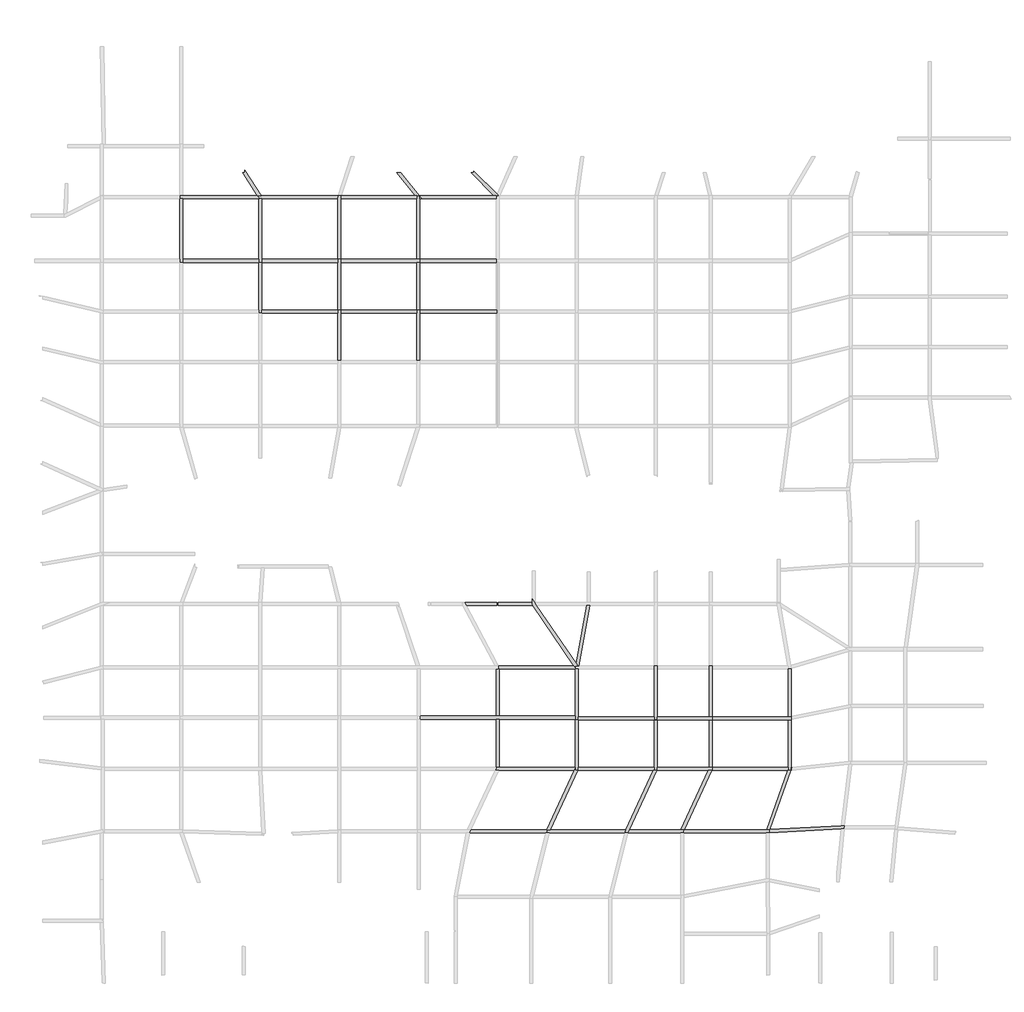
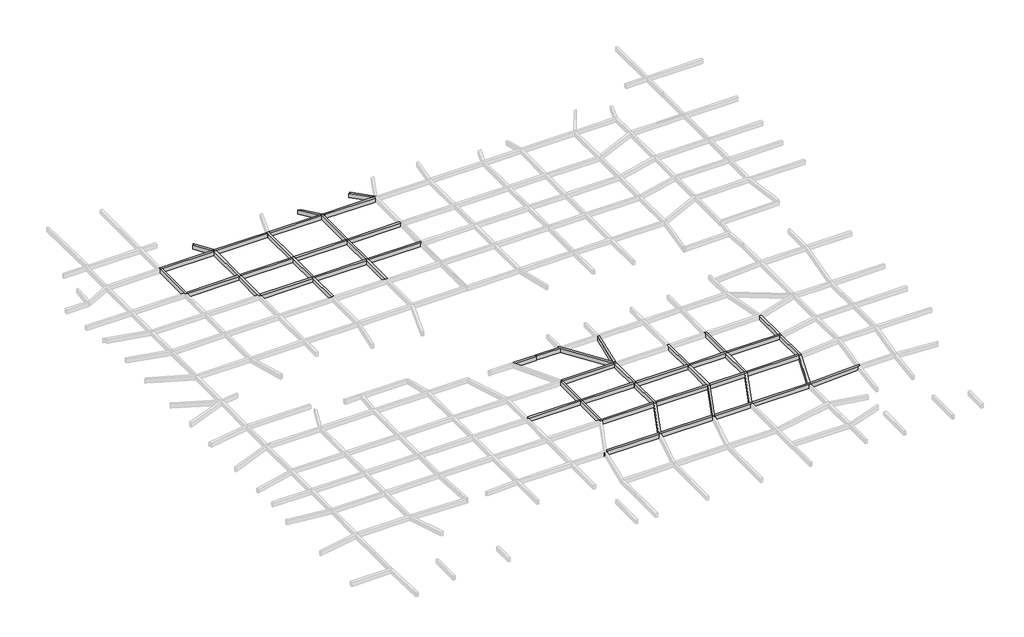
# One storey, part 9 of 15: 54 beams.
"""IFC4 building model written with IfcOpenShell, lengths in millimetres."""

from ifc_helpers import new_model, si_unit, frame, origin, place, context, project, spatial, polyline, outline, extrude, faceted_brep, element, save

model = new_model("IFC4")

# Units and contexts
model_context = context("Model", 3, world=origin())
ifc_project = project(units=[si_unit("LENGTHUNIT", "METRE", prefix="MILLI")], contexts=[model_context])

# Site, building, storey
site = spatial("IfcSite", under=ifc_project)
building = spatial("IfcBuilding", under=site)
storey = spatial("IfcBuildingStorey", under=building, Name="层高", Elevation=3300.0)

# Beams
placement = place(None, origin())
element("IfcBeam", 1, ObjectType="混凝土 - 矩形梁 : KL_beam", at=placement, inside=storey, context=model_context, shape_type="Brep", body=[
    faceted_brep([(208150.3009381, 75092.1684205, 3300.0), (208450.3009381, 75092.1684205, 3300.0), (208450.3009381, 75392.1684205, 3300.0), (208450.3009381, 80084.9176514, 3300.0), (208450.3009381, 80384.9176514, 3300.0), (208150.3009381, 80384.9176514, 3300.0), (208150.3009381, 80092.1684205, 3300.0), (208150.3009381, 75391.5531297, 3300.0), (208150.3009381, 75092.1684205, 2700.0), (208150.3009381, 80384.9176514, 2700.0), (208150.3009381, 80092.1684205, 2700.0), (208150.3009381, 75391.5531297, 2700.0), (208450.3009381, 75092.1684205, 2700.0), (208450.3009381, 80384.9176514, 2700.0), (208450.3009381, 80084.9176514, 2700.0), (208450.3009381, 75392.1684205, 2700.0)], [[[0, 1, 2, 3, 4, 5, 6, 7]], [[8, 0, 7, 6, 5, 9, 10, 11]], [[12, 8, 11, 10, 9, 13, 14, 15]], [[1, 12, 15, 14, 13, 4, 3, 2]], [[1, 0, 8, 12]], [[5, 4, 13, 9]]]),
])
element("IfcBeam", 2, ObjectType="混凝土 - 矩形梁 : KL_beam", at=placement, inside=storey, context=model_context, shape_type="Brep", body=[
    faceted_brep([(213850.3009381, 75092.1684205, 3300.0), (213850.3009381, 75392.1684205, 3300.0), (213550.3009381, 75392.1684205, 3300.0), (208450.3009381, 75392.1684205, 3300.0), (208450.3009381, 75092.1684205, 3300.0), (213549.7300619, 75092.1684205, 3300.0), (213849.7300619, 75092.1684205, 3300.0), (213850.3009381, 75092.1684205, 2700.0), (208450.3009381, 75092.1684205, 2700.0), (213549.7300619, 75092.1684205, 2700.0), (213849.7300619, 75092.1684205, 2700.0), (213850.3009381, 75392.1684205, 2700.0), (208450.3009381, 75392.1684205, 2700.0), (213550.3009381, 75392.1684205, 2700.0)], [[[0, 1, 2, 3, 4, 5, 6]], [[7, 0, 6, 5, 4, 8, 9, 10]], [[11, 7, 10, 9, 8, 12, 13]], [[1, 11, 13, 12, 3, 2]], [[4, 3, 12, 8]], [[1, 0, 7, 11]]]),
])
element("IfcBeam", 3, ObjectType="混凝土 - 矩形梁 : KL_beam", at=placement, inside=storey, context=model_context, shape_type="Brep", body=[
    faceted_brep([(213850.3009381, 80384.9176514, 3300.0), (213550.3009381, 80384.9176514, 3300.0), (213550.3009381, 80084.9176514, 3300.0), (213550.3009381, 75392.1684205, 3300.0), (213850.3009381, 75392.1684205, 3300.0), (213850.3009381, 80092.1684205, 3300.0), (213550.3009381, 80384.9176514, 2700.0), (213550.3009381, 80084.9176514, 2700.0), (213550.3009381, 75392.1684205, 2700.0), (213850.3009381, 80384.9176514, 2700.0), (213850.3009381, 80092.1684205, 2700.0), (213850.3009381, 75392.1684205, 2700.0)], [[[0, 1, 2, 3, 4, 5]], [[1, 6, 7, 8, 3, 2]], [[6, 9, 10, 11, 8, 7]], [[9, 0, 5, 4, 11, 10]], [[4, 3, 8, 11]], [[1, 0, 9, 6]]]),
])
element("IfcBeam", 4, ObjectType="混凝土 - 矩形梁 : KL_beam", at=placement, inside=storey, context=model_context, shape_type="Brep", body=[
    faceted_brep([(200361.325629, 75091.5531297, 3300.0), (200661.325629, 75091.5531297, 3300.0), (200661.325629, 75391.5531297, 3300.0), (200661.325629, 80092.1684205, 3300.0), (200361.325629, 80092.1684205, 3300.0), (200361.325629, 75445.2581831, 3300.0), (200361.325629, 75145.2581831, 3300.0), (200361.325629, 75091.5531297, 2700.0), (200361.325629, 80092.1684205, 2700.0), (200361.325629, 75445.2581831, 2700.0), (200361.325629, 75145.2581831, 2700.0), (200661.325629, 75091.5531297, 2700.0), (200661.325629, 80092.1684205, 2700.0), (200661.325629, 75391.5531297, 2700.0)], [[[0, 1, 2, 3, 4, 5, 6]], [[7, 0, 6, 5, 4, 8, 9, 10]], [[11, 7, 10, 9, 8, 12, 13]], [[1, 11, 13, 12, 3, 2]], [[4, 3, 12, 8]], [[1, 0, 7, 11]]]),
])
element("IfcBeam", 5, ObjectType="混凝土 - 矩形梁 : KL_beam", at=placement, inside=storey, context=model_context, shape_type="Brep", body=[
    faceted_brep([(208450.3009381, 75091.5531297, 3300.0), (208450.3009381, 75092.1684205, 3300.0), (208150.3009381, 75092.1684205, 3300.0), (208150.3009381, 75391.5531297, 3300.0), (200661.325629, 75391.5531297, 3300.0), (200661.325629, 75091.5531297, 3300.0), (208150.3009381, 75091.5531297, 3300.0), (208450.3009381, 75091.5531297, 2700.0), (200661.325629, 75091.5531297, 2700.0), (208150.3009381, 75091.5531297, 2700.0), (208450.3009381, 75092.1684205, 2700.0), (200661.325629, 75391.5531297, 2700.0), (208150.3009381, 75391.5531297, 2700.0), (208150.3009381, 75092.1684205, 2700.0)], [[[0, 1, 2, 3, 4, 5, 6]], [[7, 0, 6, 5, 8, 9]], [[10, 7, 9, 8, 11, 12, 13]], [[3, 12, 11, 4]], [[0, 7, 10, 1]], [[2, 13, 12, 3]], [[13, 2, 1, 10]], [[5, 4, 11, 8]]]),
])
element("IfcBeam", 6, ObjectType="混凝土 - 矩形梁 : KL_beam", at=placement, inside=storey, context=model_context, shape_type="Brep", body=[
    faceted_brep([(208150.3009381, 70090.9378389, 3300.0), (208395.8614772, 70090.9378389, 3300.0), (208450.3009381, 70090.9378389, 3300.0), (208450.3009381, 70390.9378389, 3300.0), (208450.3009381, 75091.5531297, 3300.0), (208150.3009381, 75091.5531297, 3300.0), (208150.3009381, 70390.9378389, 3300.0), (208450.3009381, 70090.9378389, 2700.0), (208450.3009381, 70390.9378389, 2700.0), (208450.3009381, 75091.5531297, 2700.0), (208395.8614772, 70090.9378389, 2700.0), (208150.3009381, 70090.9378389, 2700.0), (208150.3009381, 70390.9378389, 2700.0), (208150.3009381, 75091.5531297, 2700.0)], [[[0, 1, 2, 3, 4, 5, 6]], [[2, 7, 8, 9, 4, 3]], [[7, 10, 11, 12, 13, 9, 8]], [[11, 0, 6, 5, 13, 12]], [[5, 4, 9, 13]], [[2, 1, 0, 11, 10, 7]]]),
])
element("IfcBeam", 7, ObjectType="混凝土 - 矩形梁 : KL_beam", at=placement, inside=storey, context=model_context, shape_type="Brep", body=[
    faceted_brep([(200361.325629, 70090.9378389, 3300.0), (200607.1105063, 70090.9378389, 3300.0), (200661.325629, 70090.9378389, 3300.0), (200661.325629, 70390.9378389, 3300.0), (200661.325629, 75091.5531297, 3300.0), (200361.325629, 75091.5531297, 3300.0), (200361.325629, 70390.9378389, 3300.0), (200361.325629, 70274.0247745, 3300.0), (200361.325629, 70090.9378389, 2700.0), (200361.325629, 75091.5531297, 2700.0), (200361.325629, 70390.9378389, 2700.0), (200361.325629, 70274.0247745, 2700.0), (200661.325629, 70090.9378389, 2700.0), (200607.1105063, 70090.9378389, 2700.0), (200661.325629, 75091.5531297, 2700.0), (200661.325629, 70390.9378389, 2700.0)], [[[0, 1, 2, 3, 4, 5, 6, 7]], [[8, 0, 7, 6, 5, 9, 10, 11]], [[12, 13, 8, 11, 10, 9, 14, 15]], [[2, 12, 15, 14, 4, 3]], [[5, 4, 14, 9]], [[2, 1, 0, 8, 13, 12]]]),
])
element("IfcBeam", 8, ObjectType="混凝土 - 矩形梁 : KL_beam", at=placement, inside=storey, context=model_context, shape_type="Brep", body=[
    faceted_brep([(208150.3009381, 70090.9378389, 3300.0), (208150.3009381, 70390.9378389, 3300.0), (200661.325629, 70390.9378389, 3300.0), (200661.325629, 70090.9378389, 3300.0), (208064.8481015, 70090.9378389, 3300.0), (208150.3009381, 70090.9378389, 2700.0), (200661.325629, 70090.9378389, 2700.0), (208064.8481015, 70090.9378389, 2700.0), (208150.3009381, 70390.9378389, 2700.0), (200661.325629, 70390.9378389, 2700.0)], [[[0, 1, 2, 3, 4]], [[5, 0, 4, 3, 6, 7]], [[8, 5, 7, 6, 9]], [[1, 8, 9, 2]], [[1, 0, 5, 8]], [[3, 2, 9, 6]]]),
])
element("IfcBeam", 9, ObjectType="混凝土 - 矩形梁 : KL_beam", at=placement, inside=storey, context=model_context, shape_type="Brep", body=[
    faceted_brep([(208450.3009381, 70390.9378389, 2700.0), (208450.3009381, 70390.9378389, 3300.0), (213549.7300619, 70390.9378389, 3300.0), (213849.7300619, 70390.9378389, 3300.0), (213849.7300619, 70390.9378389, 2700.0), (213549.7300619, 70390.9378389, 2700.0), (208450.3009381, 70090.9378389, 3300.0), (208450.3009381, 70090.9378389, 2700.0), (213849.7300619, 70092.1684205, 3300.0), (213849.7300619, 70090.9378389, 3300.0), (213849.7300619, 70090.9378389, 2700.0), (213849.7300619, 70092.1684205, 2700.0), (213464.2379642, 70090.9378389, 3300.0), (213794.9360409, 70090.9378389, 3300.0), (213464.2379642, 70090.9378389, 2700.0), (213794.9360409, 70090.9378389, 2700.0)], [[[0, 1, 2, 3, 4, 5]], [[6, 1, 0, 7]], [[3, 8, 9, 10, 11, 4]], [[1, 6, 12, 13, 9, 8, 3, 2]], [[6, 7, 14, 15, 10, 9, 13, 12]], [[7, 0, 5, 4, 11, 10, 15, 14]]]),
])
element("IfcBeam", 10, ObjectType="混凝土 - 矩形梁 : KL_beam", at=placement, inside=storey, context=model_context, shape_type="Brep", body=[
    faceted_brep([(213849.7300619, 75092.1684205, 3300.0), (213549.7300619, 75092.1684205, 3300.0), (213549.7300619, 70390.9378389, 3300.0), (213849.7300619, 70390.9378389, 3300.0), (213849.7300619, 70392.1684205, 3300.0), (213849.7300619, 75092.1684205, 2700.0), (213849.7300619, 70390.9378389, 2700.0), (213849.7300619, 70392.1684205, 2700.0), (213549.7300619, 75092.1684205, 2700.0), (213549.7300619, 70390.9378389, 2700.0)], [[[0, 1, 2, 3, 4]], [[5, 0, 4, 3, 6, 7]], [[8, 5, 7, 6, 9]], [[1, 8, 9, 2]], [[1, 0, 5, 8]], [[3, 2, 9, 6]]]),
])
element("IfcBeam", 11, ObjectType="混凝土 - 矩形梁 : KL_beam", at=placement, inside=storey, context=model_context, shape_type="Brep", body=[
    faceted_brep([(221650.3009384, 75092.1684205, 3300.0), (221650.3009384, 75119.2786858, 3300.0), (221650.3009384, 75392.1684205, 3300.0), (221485.3991695, 75392.1684205, 3300.0), (221350.3009384, 75392.1684205, 3300.0), (213850.3009381, 75392.1684205, 3300.0), (213850.3009381, 75092.1684205, 3300.0), (221350.3009384, 75092.1684205, 3300.0), (221650.3009384, 75092.1684205, 2700.0), (213850.3009381, 75092.1684205, 2700.0), (221350.3009384, 75092.1684205, 2700.0), (221650.3009384, 75392.1684205, 2700.0), (221650.3009384, 75119.2786858, 2700.0), (213850.3009381, 75392.1684205, 2700.0), (221350.3009384, 75392.1684205, 2700.0), (221485.3991695, 75392.1684205, 2700.0)], [[[0, 1, 2, 3, 4, 5, 6, 7]], [[8, 0, 7, 6, 9, 10]], [[11, 12, 8, 10, 9, 13, 14, 15]], [[2, 11, 15, 14, 13, 5, 4, 3]], [[6, 5, 13, 9]], [[2, 1, 0, 8, 12, 11]]]),
])
element("IfcBeam", 12, ObjectType="混凝土 - 矩形梁 : KL_beam", at=placement, inside=storey, context=model_context, shape_type="Brep", body=[
    faceted_brep([(221350.3009384, 70092.1684205, 3300.0), (221606.4676056, 70092.1684205, 3300.0), (221650.3009384, 70092.1684205, 3300.0), (221650.3009384, 70106.4638205, 3300.0), (221650.3009384, 70216.5015374, 3300.0), (221650.3009384, 70407.9697272, 3300.0), (221650.3009384, 75092.1684205, 3300.0), (221350.3009384, 75092.1684205, 3300.0), (221350.3009384, 70392.1684205, 3300.0), (221350.3009384, 70092.1684205, 2700.0), (221350.3009384, 75092.1684205, 2700.0), (221350.3009384, 70392.1684205, 2700.0), (221650.3009384, 70092.1684205, 2700.0), (221606.4676056, 70092.1684205, 2700.0), (221650.3009384, 75092.1684205, 2700.0), (221650.3009384, 70407.9697272, 2700.0), (221650.3009384, 70216.5015374, 2700.0), (221650.3009384, 70106.4638205, 2700.0)], [[[0, 1, 2, 3, 4, 5, 6, 7, 8]], [[9, 0, 8, 7, 10, 11]], [[12, 13, 9, 11, 10, 14, 15, 16, 17]], [[2, 12, 17, 16, 15, 14, 6, 5, 4, 3]], [[7, 6, 14, 10]], [[2, 1, 0, 9, 13, 12]]]),
])
element("IfcBeam", 13, ObjectType="混凝土 - 矩形梁 : KL_beam", at=placement, inside=storey, context=model_context, shape_type="Brep", body=[
    faceted_brep([(213849.7300619, 70392.1684205, 3300.0), (213849.7300619, 70390.9378389, 3300.0), (213849.7300619, 70092.1684205, 3300.0), (221288.3700133, 70092.1684205, 3300.0), (221350.3009384, 70092.1684205, 3300.0), (221350.3009384, 70392.1684205, 3300.0), (213849.7300619, 70392.1684205, 2700.0), (221350.3009384, 70392.1684205, 2700.0), (213849.7300619, 70092.1684205, 2700.0), (213849.7300619, 70390.9378389, 2700.0), (221350.3009384, 70092.1684205, 2700.0), (221288.3700133, 70092.1684205, 2700.0)], [[[0, 1, 2, 3, 4, 5]], [[6, 0, 5, 7]], [[8, 9, 6, 7, 10, 11]], [[2, 8, 11, 10, 4, 3]], [[8, 2, 1, 0, 6, 9]], [[5, 4, 10, 7]]]),
])
element("IfcBeam", 14, ObjectType="混凝土 - 矩形梁 : KL_beam", at=placement, inside=storey, context=model_context, shape_type="Brep", body=[
    faceted_brep([(205522.0572974, 63928.0448871, 3300.0), (205661.9495948, 64228.0448871, 3300.0), (208395.8614772, 70090.9378389, 3300.0), (208150.3009381, 70090.9378389, 3300.0), (208064.8481015, 70090.9378389, 3300.0), (205337.522131, 64242.1684205, 3300.0), (205250.1649613, 64054.8303656, 3300.0), (205491.7692821, 63942.1684205, 3300.0), (208064.8481015, 70090.9378389, 2700.0), (205337.522131, 64242.1684205, 2700.0), (205250.1649613, 64054.8303656, 2700.0), (208395.8614772, 70090.9378389, 2700.0), (205661.9495948, 64228.0448871, 2700.0), (205522.0572974, 63928.0448871, 2700.0), (205491.7692821, 63942.1684205, 2700.0), (208150.3009381, 70090.9378389, 2700.0)], [[[0, 1, 2, 3, 4, 5, 6, 7]], [[6, 5, 4, 8, 9, 10]], [[11, 12, 13, 14, 10, 9, 8, 15]], [[2, 1, 0, 13, 12, 11]], [[2, 11, 15, 8, 4, 3]], [[0, 7, 6, 10, 14, 13]]]),
])
element("IfcBeam", 15, ObjectType="混凝土 - 矩形梁 : KL_beam", at=placement, inside=storey, context=model_context, shape_type="Brep", body=[
    faceted_brep([(210936.491926, 63928.0448871, 3300.0), (210945.3598239, 63947.1643462, 3300.0), (211075.6365195, 64228.0448871, 3300.0), (210744.9384428, 64228.0448871, 3300.0), (205661.9495948, 64228.0448871, 3300.0), (205522.0572974, 63928.0448871, 3300.0), (205546.7541217, 63928.0448871, 3300.0), (210741.9011747, 63928.0448871, 3300.0), (210936.491926, 63928.0448871, 2700.0), (205522.0572974, 63928.0448871, 2700.0), (205546.7541217, 63928.0448871, 2700.0), (210741.9011747, 63928.0448871, 2700.0), (211075.6365195, 64228.0448871, 2700.0), (210945.3598239, 63947.1643462, 2700.0), (205661.9495948, 64228.0448871, 2700.0), (210744.9384428, 64228.0448871, 2700.0)], [[[0, 1, 2, 3, 4, 5, 6, 7]], [[8, 0, 7, 6, 5, 9, 10, 11]], [[12, 13, 8, 11, 10, 9, 14, 15]], [[2, 12, 15, 14, 4, 3]], [[5, 4, 14, 9]], [[2, 1, 0, 8, 13, 12]]]),
])
element("IfcBeam", 16, ObjectType="混凝土 - 矩形梁 : KL_beam", at=placement, inside=storey, context=model_context, shape_type="Brep", body=[
    faceted_brep([(210744.9384428, 64228.0448871, 3300.0), (211075.6365195, 64228.0448871, 3300.0), (211084.5044173, 64247.1643462, 3300.0), (213794.9360409, 70090.9378389, 3300.0), (213464.2379642, 70090.9378389, 3300.0), (211075.6365195, 64228.0448871, 2700.0), (211084.5044173, 64247.1643462, 2700.0), (213794.9360409, 70090.9378389, 2700.0), (210744.9384428, 64228.0448871, 2700.0), (213464.2379642, 70090.9378389, 2700.0)], [[[0, 1, 2, 3, 4]], [[1, 5, 6, 7, 3, 2]], [[5, 8, 9, 7, 6]], [[8, 0, 4, 9]], [[1, 0, 8, 5]], [[3, 7, 9, 4]]]),
])
element("IfcBeam", 17, ObjectType="混凝土 - 矩形梁 : KL_beam", at=placement, inside=storey, context=model_context, shape_type="Brep", body=[
    faceted_brep([(211084.5044173, 64247.1643462, 3300.0), (211075.6365195, 64228.0448871, 3300.0), (210945.3598239, 63947.1643462, 3300.0), (211041.9011747, 63947.1643462, 3300.0), (219183.8949524, 63947.1643462, 3300.0), (219483.8949524, 63947.1643462, 3300.0), (219483.8949524, 63954.8196612, 3300.0), (219483.8949524, 64247.1643462, 3300.0), (219329.9670642, 64247.1643462, 3300.0), (219227.7282852, 64247.1643462, 3300.0), (219483.8949524, 64247.1643462, 2700.0), (219329.9670642, 64247.1643462, 2700.0), (219227.7282852, 64247.1643462, 2700.0), (211084.5044173, 64247.1643462, 2700.0), (210945.3598239, 63947.1643462, 2700.0), (211075.6365195, 64228.0448871, 2700.0), (219483.8949524, 63954.8196612, 2700.0), (219483.8949524, 63947.1643462, 2700.0), (219183.8949524, 63947.1643462, 2700.0), (211041.9011747, 63947.1643462, 2700.0)], [[[0, 1, 2, 3, 4, 5, 6, 7, 8, 9]], [[7, 10, 11, 12, 13, 0, 9, 8]], [[14, 15, 13, 12, 11, 10, 16, 17, 18, 19]], [[2, 14, 19, 18, 17, 5, 4, 3]], [[0, 13, 15, 14, 2, 1]], [[7, 6, 5, 17, 16, 10]]]),
])
element("IfcBeam", 18, ObjectType="混凝土 - 矩形梁 : KL_beam", at=placement, inside=storey, context=model_context, shape_type="Brep", body=[
    faceted_brep([(205337.522131, 64242.1684205, 3300.0), (197894.9093254, 64242.1684205, 3300.0), (197564.2230667, 64242.1684205, 3300.0), (197564.2230667, 63942.1684205, 3300.0), (197777.200788, 63942.1684205, 3300.0), (205241.0914253, 63942.1684205, 3300.0), (205491.7692821, 63942.1684205, 3300.0), (205250.1649613, 64054.8303656, 3300.0), (205330.9362192, 64228.0448871, 3300.0), (197564.2230667, 63942.1684205, 2700.0), (197777.200788, 63942.1684205, 2700.0), (205241.0914253, 63942.1684205, 2700.0), (205491.7692821, 63942.1684205, 2700.0), (197564.2230667, 64242.1684205, 2700.0), (197894.9093254, 64242.1684205, 2700.0), (205337.522131, 64242.1684205, 2700.0), (205330.9362192, 64228.0448871, 2700.0), (205250.1649613, 64054.8303656, 2700.0)], [[[0, 1, 2, 3, 4, 5, 6, 7, 8]], [[6, 5, 4, 3, 9, 10, 11, 12]], [[12, 11, 10, 9, 13, 14, 15, 16, 17]], [[2, 1, 0, 15, 14, 13]], [[7, 17, 16, 15, 0, 8]], [[17, 7, 6, 12]], [[2, 13, 9, 3]]]),
])
element("IfcBeam", 19, ObjectType="混凝土 - 矩形梁 : KL_beam", at=placement, inside=storey, context=model_context, shape_type="Brep", body=[
    faceted_brep([(200361.325629, 70274.0247745, 3300.0), (200276.4242476, 70090.9378389, 3300.0), (197564.2230667, 64242.1684205, 3300.0), (197894.9093254, 64242.1684205, 3300.0), (200607.1105063, 70090.9378389, 3300.0), (200361.325629, 70090.9378389, 3300.0), (200361.325629, 70274.0247745, 2700.0), (200276.4242476, 70090.9378389, 2700.0), (197564.2230667, 64242.1684205, 2700.0), (200361.325629, 70090.9378389, 2700.0), (200607.1105063, 70090.9378389, 2700.0), (197894.9093254, 64242.1684205, 2700.0)], [[[0, 1, 2, 3, 4, 5]], [[2, 1, 0, 6, 7, 8]], [[8, 7, 6, 9, 10, 11]], [[10, 4, 3, 11]], [[5, 9, 6, 0]], [[9, 5, 4, 10]], [[3, 2, 8, 11]]]),
])
element("IfcBeam", 20, ObjectType="混凝土 - 矩形梁 : KL_beam", at=placement, inside=storey, context=model_context, shape_type="Brep", body=[
    faceted_brep([(192604.8334695, 70390.9378389, 3300.0), (192464.0250307, 70090.9378389, 3300.0), (192795.4266246, 70090.9378389, 3300.0), (200276.4242476, 70090.9378389, 3300.0), (200361.325629, 70274.0247745, 3300.0), (200361.325629, 70390.9378389, 3300.0), (192850.1300471, 70390.9378389, 3300.0), (200361.325629, 70390.9378389, 2700.0), (192850.1300471, 70390.9378389, 2700.0), (192604.8334695, 70390.9378389, 2700.0), (192464.0250307, 70090.9378389, 2700.0), (200361.325629, 70274.0247745, 2700.0), (200276.4242476, 70090.9378389, 2700.0), (192795.4266246, 70090.9378389, 2700.0)], [[[0, 1, 2, 3, 4, 5, 6]], [[5, 7, 8, 9, 0, 6]], [[10, 9, 8, 7, 11, 12, 13]], [[1, 10, 13, 12, 3, 2]], [[7, 5, 4, 11]], [[4, 3, 12, 11]], [[1, 0, 9, 10]]]),
])
element("IfcBeam", 21, ObjectType="混凝土 - 矩形梁 : KL_beam", at=placement, inside=storey, context=model_context, shape_type="Brep", body=[
    faceted_brep([(189578.0296218, 63942.1684205, 3300.0), (189632.1700876, 63942.1684205, 3300.0), (189937.7850961, 63942.1684205, 3300.0), (197468.0166992, 63942.1684205, 3300.0), (197564.2230667, 63942.1684205, 3300.0), (197564.2230667, 64242.1684205, 3300.0), (190050.2396546, 64242.1684205, 3300.0), (189910.8814312, 63945.2581831, 3300.0), (189579.4798373, 63945.2581831, 3300.0), (197564.2230667, 64242.1684205, 2700.0), (190050.2396546, 64242.1684205, 2700.0), (197564.2230667, 63942.1684205, 2700.0), (197468.0166992, 63942.1684205, 2700.0), (189937.7850961, 63942.1684205, 2700.0), (189632.1700876, 63942.1684205, 2700.0), (189578.0296218, 63942.1684205, 2700.0), (189579.4798373, 63945.2581831, 2700.0), (189910.8814312, 63945.2581831, 2700.0)], [[[0, 1, 2, 3, 4, 5, 6, 7, 8]], [[5, 9, 10, 6]], [[11, 12, 13, 14, 15, 16, 17, 10, 9]], [[0, 15, 14, 13, 12, 11, 4, 3, 2, 1]], [[15, 0, 8, 16]], [[5, 4, 11, 9]], [[7, 17, 16, 8]], [[17, 7, 6, 10]]]),
])
element("IfcBeam", 22, ObjectType="混凝土 - 矩形梁 : KL_beam", at=placement, inside=storey, context=model_context, shape_type="Brep", body=[
    faceted_brep([(185065.5848537, 75445.2581831, 3300.0), (185065.5848537, 75145.2581831, 3300.0), (192550.1300471, 75145.2581831, 3300.0), (192850.1300471, 75145.2581831, 3300.0), (200361.325629, 75145.2581831, 3300.0), (200361.325629, 75445.2581831, 3300.0), (192850.1300471, 75445.2581831, 3300.0), (192550.1300471, 75445.2581831, 3300.0), (185065.5848537, 75145.2581831, 2700.0), (192550.1300471, 75145.2581831, 2700.0), (192850.1300471, 75145.2581831, 2700.0), (200361.325629, 75145.2581831, 2700.0), (185065.5848537, 75445.2581831, 2700.0), (192550.1300471, 75445.2581831, 2700.0), (192850.1300471, 75445.2581831, 2700.0), (200361.325629, 75445.2581831, 2700.0)], [[[0, 1, 2, 3, 4, 5, 6, 7]], [[1, 8, 9, 10, 11, 4, 3, 2]], [[8, 12, 13, 14, 15, 11, 10, 9]], [[12, 0, 7, 6, 5, 15, 14, 13]], [[1, 0, 12, 8]], [[5, 4, 11, 15]]]),
])
element("IfcBeam", 23, ObjectType="混凝土 - 矩形梁 : KL_beam", at=placement, inside=storey, context=model_context, shape_type="Brep", body=[
    faceted_brep([(200361.325629, 80392.1684205, 3300.0), (200590.9130323, 80392.1684205, 3300.0), (200430.7160379, 80628.7721233, 3300.0), (196535.9381364, 86381.1826239, 3300.0), (196428.3344611, 86540.1083772, 3300.0), (196128.3344611, 86983.1947852, 3300.0), (196128.3344611, 86681.1826239, 3300.0), (196128.3344611, 86448.1008075, 3300.0), (196173.642678, 86381.1826239, 3300.0), (200228.6175739, 80392.1684205, 3300.0), (200361.325629, 80196.1646357, 3300.0), (200361.325629, 80196.1646357, 2700.0), (196128.3344611, 86448.1008075, 2700.0), (196173.642678, 86381.1826239, 2700.0), (200228.6175739, 80392.1684205, 2700.0), (200590.9130323, 80392.1684205, 2700.0), (200361.325629, 80392.1684205, 2700.0), (196128.3344611, 86681.1826239, 2700.0), (196128.3344611, 86983.1947852, 2700.0), (196428.3344611, 86540.1083772, 2700.0), (196535.9381364, 86381.1826239, 2700.0), (200430.7160379, 80628.7721233, 2700.0)], [[[0, 1, 2, 3, 4, 5, 6, 7, 8, 9, 10]], [[11, 10, 9, 8, 7, 12, 13, 14]], [[15, 16, 11, 14, 13, 12, 17, 18, 19, 20, 21]], [[1, 15, 21, 20, 19, 18, 5, 4, 3, 2]], [[0, 16, 15, 1]], [[16, 0, 10, 11]], [[7, 6, 5, 18, 17, 12]]]),
])
element("IfcBeam", 24, ObjectType="混凝土 - 矩形梁 : KL_beam", at=placement, inside=storey, context=model_context, shape_type="Brep", body=[
    faceted_brep([(200361.325629, 80092.1684205, 3300.0), (200361.325629, 80196.1646357, 3300.0), (200228.6175739, 80392.1684205, 3300.0), (192790.538789, 80392.1684205, 3300.0), (192790.538789, 80092.1684205, 3300.0), (192850.1300471, 80092.1684205, 3300.0), (200228.6175739, 80392.1684205, 2700.0), (192790.538789, 80392.1684205, 2700.0), (200361.325629, 80196.1646357, 2700.0), (200361.325629, 80092.1684205, 2700.0), (192850.1300471, 80092.1684205, 2700.0), (192790.538789, 80092.1684205, 2700.0)], [[[0, 1, 2, 3, 4, 5]], [[2, 6, 7, 3]], [[8, 9, 10, 11, 7, 6]], [[9, 0, 5, 4, 11, 10]], [[0, 9, 8, 1]], [[2, 1, 8, 6]], [[4, 3, 7, 11]]]),
])
element("IfcBeam", 25, ObjectType="混凝土 - 矩形梁 : KL_beam", at=placement, inside=storey, context=model_context, shape_type="Brep", body=[
    faceted_brep([(185050.3009381, 115492.1448334, 3300.0), (184750.3009381, 115492.1448334, 3300.0), (184750.3009381, 115192.1448334, 3300.0), (184750.3009381, 110492.1448334, 3300.0), (185050.3009381, 110492.1448334, 3300.0), (185050.3009381, 115192.1448334, 3300.0), (184750.3009381, 115492.1448334, 2700.0), (184750.3009381, 115192.1448334, 2700.0), (184750.3009381, 110492.1448334, 2700.0), (185050.3009381, 115492.1448334, 2700.0), (185050.3009381, 115192.1448334, 2700.0), (185050.3009381, 110492.1448334, 2700.0)], [[[0, 1, 2, 3, 4, 5]], [[1, 6, 7, 8, 3, 2]], [[6, 9, 10, 11, 8, 7]], [[9, 0, 5, 4, 11, 10]], [[4, 3, 8, 11]], [[1, 0, 9, 6]]]),
])
element("IfcBeam", 26, ObjectType="混凝土 - 矩形梁 : KL_beam", at=placement, inside=storey, context=model_context, shape_type="Brep", body=[
    faceted_brep([(177250.3009381, 115492.1448334, 3300.0), (176950.3009381, 115492.1448334, 3300.0), (176950.3009381, 115192.1448334, 3300.0), (176950.3009381, 110492.1448334, 3300.0), (177250.3009381, 110492.1448334, 3300.0), (177250.3009381, 115192.1448334, 3300.0), (176950.3009381, 115492.1448334, 2700.0), (176950.3009381, 115192.1448334, 2700.0), (176950.3009381, 110492.1448334, 2700.0), (177250.3009381, 115492.1448334, 2700.0), (177250.3009381, 115192.1448334, 2700.0), (177250.3009381, 110492.1448334, 2700.0)], [[[0, 1, 2, 3, 4, 5]], [[1, 6, 7, 8, 3, 2]], [[6, 9, 10, 11, 8, 7]], [[9, 0, 5, 4, 11, 10]], [[4, 3, 8, 11]], [[1, 0, 9, 6]]]),
])
element("IfcBeam", 27, ObjectType="混凝土 - 矩形梁 : KL_beam", at=placement, inside=storey, context=model_context, shape_type="SweptSolid", body=[
    extrude(outline(polyline([(184750.3009381, 115492.1448334), (184750.3009381, 115192.1448334), (177250.3009381, 115192.1448334), (177250.3009381, 115492.1448334), (184750.3009381, 115492.1448334)])), frame((0.0, 0.0, 2700.0), z_axis=(0.0, 0.0, 1.0), x_axis=(1.0, 0.0, 0.0)), (0.0, 0.0, 1.0), 600.0),
])
element("IfcBeam", 28, ObjectType="混凝土 - 矩形梁 : KL_beam", at=placement, inside=storey, context=model_context, shape_type="Brep", body=[
    faceted_brep([(177250.3009381, 120492.1448334, 3300.0), (176950.3009381, 120492.1448334, 3300.0), (176950.3009381, 120192.1448334, 3300.0), (176950.3009381, 115492.1448334, 3300.0), (177250.3009381, 115492.1448334, 3300.0), (177250.3009381, 120192.1448334, 3300.0), (176950.3009381, 120492.1448334, 2700.0), (176950.3009381, 120192.1448334, 2700.0), (176950.3009381, 115492.1448334, 2700.0), (177250.3009381, 120492.1448334, 2700.0), (177250.3009381, 120192.1448334, 2700.0), (177250.3009381, 115492.1448334, 2700.0)], [[[0, 1, 2, 3, 4, 5]], [[1, 6, 7, 8, 3, 2]], [[6, 9, 10, 11, 8, 7]], [[9, 0, 5, 4, 11, 10]], [[4, 3, 8, 11]], [[1, 0, 9, 6]]]),
])
element("IfcBeam", 29, ObjectType="混凝土 - 矩形梁 : KL_beam", at=placement, inside=storey, context=model_context, shape_type="Brep", body=[
    faceted_brep([(185050.3009381, 120192.1448334, 3300.0), (185050.3009381, 120492.1448334, 3300.0), (184750.3009381, 120492.1448334, 3300.0), (177250.3009381, 120492.1448334, 3300.0), (177250.3009381, 120192.1448334, 3300.0), (184750.3009381, 120192.1448334, 3300.0), (185050.3009381, 120192.1448334, 2700.0), (177250.3009381, 120192.1448334, 2700.0), (184750.3009381, 120192.1448334, 2700.0), (185050.3009381, 120492.1448334, 2700.0), (177250.3009381, 120492.1448334, 2700.0), (184750.3009381, 120492.1448334, 2700.0)], [[[0, 1, 2, 3, 4, 5]], [[6, 0, 5, 4, 7, 8]], [[9, 6, 8, 7, 10, 11]], [[1, 9, 11, 10, 3, 2]], [[4, 3, 10, 7]], [[1, 0, 6, 9]]]),
])
element("IfcBeam", 30, ObjectType="混凝土 - 矩形梁 : KL_beam", at=placement, inside=storey, context=model_context, shape_type="SweptSolid", body=[
    extrude(outline(polyline([(185050.3009381, 115492.1448334), (184750.3009381, 115492.1448334), (184750.3009381, 120192.1448334), (185050.3009381, 120192.1448334), (185050.3009381, 115492.1448334)])), frame((0.0, 0.0, 2700.0), z_axis=(0.0, 0.0, 1.0), x_axis=(1.0, 0.0, 0.0)), (0.0, 0.0, 1.0), 600.0),
])
element("IfcBeam", 31, ObjectType="混凝土 - 矩形梁 : KL_beam", at=placement, inside=storey, context=model_context, shape_type="Brep", body=[
    faceted_brep([(177250.3009381, 126792.1448334, 3300.0), (176991.4064824, 126792.1448334, 3300.0), (176950.3009381, 126792.1448334, 3300.0), (176950.3009381, 126665.9608383, 3300.0), (176950.3009381, 126492.1448334, 3300.0), (176950.3009381, 120492.1448334, 3300.0), (177250.3009381, 120492.1448334, 3300.0), (177250.3009381, 126492.1448334, 3300.0), (176950.3009381, 126792.1448334, 2700.0), (176950.3009381, 126665.9608383, 2700.0), (176950.3009381, 126492.1448334, 2700.0), (176950.3009381, 120492.1448334, 2700.0), (176991.4064824, 126792.1448334, 2700.0), (177250.3009381, 126792.1448334, 2700.0), (177250.3009381, 126492.1448334, 2700.0), (177250.3009381, 120492.1448334, 2700.0)], [[[0, 1, 2, 3, 4, 5, 6, 7]], [[2, 8, 9, 10, 11, 5, 4, 3]], [[8, 12, 13, 14, 15, 11, 10, 9]], [[13, 0, 7, 6, 15, 14]], [[6, 5, 11, 15]], [[2, 1, 0, 13, 12, 8]]]),
])
element("IfcBeam", 32, ObjectType="混凝土 - 矩形梁 : KL_beam", at=placement, inside=storey, context=model_context, shape_type="Brep", body=[
    faceted_brep([(185050.3009381, 126792.1448334, 3300.0), (184971.847268, 126792.1448334, 3300.0), (184750.3009381, 126792.1448334, 3300.0), (184750.3009381, 126492.1448334, 3300.0), (184750.3009381, 120492.1448334, 3300.0), (185050.3009381, 120492.1448334, 3300.0), (185050.3009381, 126492.1448334, 3300.0), (185050.3009381, 126695.2626192, 3300.0), (184750.3009381, 126792.1448334, 2700.0), (184750.3009381, 126492.1448334, 2700.0), (184750.3009381, 120492.1448334, 2700.0), (184971.847268, 126792.1448334, 2700.0), (185050.3009381, 126792.1448334, 2700.0), (185050.3009381, 126695.2626192, 2700.0), (185050.3009381, 126492.1448334, 2700.0), (185050.3009381, 120492.1448334, 2700.0)], [[[0, 1, 2, 3, 4, 5, 6, 7]], [[2, 8, 9, 10, 4, 3]], [[8, 11, 12, 13, 14, 15, 10, 9]], [[12, 0, 7, 6, 5, 15, 14, 13]], [[5, 4, 10, 15]], [[2, 1, 0, 12, 11, 8]]]),
])
element("IfcBeam", 33, ObjectType="混凝土 - 矩形梁 : KL_beam", at=placement, inside=storey, context=model_context, shape_type="Brep", body=[
    faceted_brep([(177250.3009381, 126792.1448334, 3300.0), (177250.3009381, 126492.1448334, 3300.0), (184750.3009381, 126492.1448334, 3300.0), (184750.3009381, 126792.1448334, 3300.0), (184585.8193983, 126792.1448334, 3300.0), (177306.9230278, 126792.1448334, 3300.0), (177250.3009381, 126492.1448334, 2700.0), (184750.3009381, 126492.1448334, 2700.0), (177250.3009381, 126792.1448334, 2700.0), (177306.9230278, 126792.1448334, 2700.0), (184585.8193983, 126792.1448334, 2700.0), (184750.3009381, 126792.1448334, 2700.0)], [[[0, 1, 2, 3, 4, 5]], [[1, 6, 7, 2]], [[6, 8, 9, 10, 11, 7]], [[8, 0, 5, 4, 3, 11, 10, 9]], [[1, 0, 8, 6]], [[3, 2, 7, 11]]]),
])
element("IfcBeam", 34, ObjectType="混凝土 - 矩形梁 : KL_beam", at=placement, inside=storey, context=model_context, shape_type="Brep", body=[
    faceted_brep([(183161.6670249, 129027.5312684, 3300.0), (182775.6391551, 129027.5312684, 3300.0), (184585.8193983, 126792.1448334, 3300.0), (184750.3009381, 126792.1448334, 3300.0), (184971.847268, 126792.1448334, 3300.0), (183161.6670249, 129027.5312684, 2700.0), (184971.847268, 126792.1448334, 2700.0), (182775.6391551, 129027.5312684, 2700.0), (184750.3009381, 126792.1448334, 2700.0), (184585.8193983, 126792.1448334, 2700.0)], [[[0, 1, 2, 3, 4]], [[5, 0, 4, 6]], [[7, 5, 6, 8, 9]], [[1, 7, 9, 2]], [[1, 0, 5, 7]], [[2, 9, 8, 6, 4, 3]]]),
    faceted_brep([(185050.3009381, 126492.1448334, 3300.0), (185050.3009381, 126695.2626192, 3300.0), (185050.3009381, 126695.2626192, 2700.0), (185050.3009381, 126492.1448334, 2700.0), (185214.782478, 126492.1448334, 2700.0), (185214.782478, 126492.1448334, 3300.0)], [[[0, 1, 2, 3]], [[4, 5, 0, 3]], [[5, 1, 0]], [[1, 5, 4, 2]], [[2, 4, 3]]]),
])
element("IfcBeam", 35, ObjectType="混凝土 - 矩形梁 : KL_beam", at=placement, inside=storey, context=model_context, shape_type="Brep", body=[
    faceted_brep([(169022.9398412, 126792.1448334, 3300.0), (169219.1792514, 126492.1448334, 3300.0), (169450.3009381, 126492.1448334, 3300.0), (176893.6788484, 126492.1448334, 3300.0), (176950.3009381, 126665.9608383, 3300.0), (176950.3009381, 126792.1448334, 3300.0), (169381.4226248, 126792.1448334, 3300.0), (169219.1792514, 126492.1448334, 2700.0), (169450.3009381, 126492.1448334, 2700.0), (176893.6788484, 126492.1448334, 2700.0), (169022.9398412, 126792.1448334, 2700.0), (169381.4226248, 126792.1448334, 2700.0), (176950.3009381, 126792.1448334, 2700.0), (176950.3009381, 126665.9608383, 2700.0)], [[[0, 1, 2, 3, 4, 5, 6]], [[1, 7, 8, 9, 3, 2]], [[7, 10, 11, 12, 13, 9, 8]], [[5, 12, 11, 10, 0, 6]], [[12, 5, 4, 13]], [[4, 3, 9, 13]], [[1, 0, 10, 7]]]),
])
element("IfcBeam", 36, ObjectType="混凝土 - 矩形梁 : KL_beam", at=placement, inside=storey, context=model_context, shape_type="SweptSolid", body=[
    extrude(outline(polyline([(167560.7034552, 129027.5312684), (167760.6969649, 129027.5312684), (167760.6969649, 129269.8209394), (169381.4226248, 126792.1448334), (169022.9398412, 126792.1448334), (167560.7034552, 129027.5312684)])), frame((0.0, 0.0, 2700.0), z_axis=(0.0, 0.0, 1.0), x_axis=(1.0, 0.0, 0.0)), (0.0, 0.0, 1.0), 600.0),
])
element("IfcBeam", 37, ObjectType="混凝土 - 矩形梁 : KL_beam", at=placement, inside=storey, context=model_context, shape_type="Brep", body=[
    faceted_brep([(169219.1792514, 126492.1448334, 3300.0), (169022.9398412, 126792.1448334, 3300.0), (161650.3009383, 126792.1448334, 3300.0), (161350.3009383, 126792.1448334, 3300.0), (161350.3009383, 126492.1448334, 3300.0), (161650.3009383, 126492.1448334, 3300.0), (169150.3009381, 126492.1448334, 3300.0), (169219.1792514, 126492.1448334, 2700.0), (161350.3009383, 126492.1448334, 2700.0), (161650.3009383, 126492.1448334, 2700.0), (169150.3009381, 126492.1448334, 2700.0), (169022.9398412, 126792.1448334, 2700.0), (161350.3009383, 126792.1448334, 2700.0), (161650.3009383, 126792.1448334, 2700.0)], [[[0, 1, 2, 3, 4, 5, 6]], [[7, 0, 6, 5, 4, 8, 9, 10]], [[11, 7, 10, 9, 8, 12, 13]], [[1, 11, 13, 12, 3, 2]], [[1, 0, 7, 11]], [[4, 3, 12, 8]]]),
])
element("IfcBeam", 38, ObjectType="混凝土 - 矩形梁 : KL_beam", at=placement, inside=storey, context=model_context, shape_type="Brep", body=[
    faceted_brep([(161350.3009383, 120192.1448334, 3300.0), (161650.3009383, 120192.1448334, 3300.0), (161650.3009383, 120492.1448334, 3300.0), (161650.3009383, 126492.1448334, 3300.0), (161350.3009383, 126492.1448334, 3300.0), (161350.3009383, 120492.1448334, 3300.0), (161350.3009383, 120192.1448334, 2700.0), (161350.3009383, 126492.1448334, 2700.0), (161350.3009383, 120492.1448334, 2700.0), (161650.3009383, 120192.1448334, 2700.0), (161650.3009383, 126492.1448334, 2700.0), (161650.3009383, 120492.1448334, 2700.0)], [[[0, 1, 2, 3, 4, 5]], [[6, 0, 5, 4, 7, 8]], [[9, 6, 8, 7, 10, 11]], [[1, 9, 11, 10, 3, 2]], [[4, 3, 10, 7]], [[1, 0, 6, 9]]]),
])
element("IfcBeam", 39, ObjectType="混凝土 - 矩形梁 : KL_beam", at=placement, inside=storey, context=model_context, shape_type="Brep", body=[
    faceted_brep([(169450.3009381, 126492.1448334, 3300.0), (169219.1792514, 126492.1448334, 3300.0), (169150.3009381, 126492.1448334, 3300.0), (169150.3009381, 120492.1448334, 3300.0), (169150.3009381, 120192.1448334, 3300.0), (169450.3009381, 120192.1448334, 3300.0), (169450.3009381, 120492.1448334, 3300.0), (169450.3009381, 126492.1448334, 2700.0), (169450.3009381, 120192.1448334, 2700.0), (169450.3009381, 120492.1448334, 2700.0), (169150.3009381, 126492.1448334, 2700.0), (169219.1792514, 126492.1448334, 2700.0), (169150.3009381, 120192.1448334, 2700.0), (169150.3009381, 120492.1448334, 2700.0)], [[[0, 1, 2, 3, 4, 5, 6]], [[7, 0, 6, 5, 8, 9]], [[10, 11, 7, 9, 8, 12, 13]], [[12, 4, 3, 2, 10, 13]], [[0, 7, 11, 10, 2, 1]], [[5, 4, 12, 8]]]),
])
element("IfcBeam", 40, ObjectType="混凝土 - 矩形梁 : KL_beam", at=placement, inside=storey, context=model_context, shape_type="Brep", body=[
    faceted_brep([(169150.3009381, 115192.1448334, 3300.0), (169450.3009381, 115192.1448334, 3300.0), (169450.3009381, 115492.1448334, 3300.0), (169450.3009381, 120192.1448334, 3300.0), (169150.3009381, 120192.1448334, 3300.0), (169150.3009381, 115492.1448334, 3300.0), (169450.3009381, 115192.1448334, 2700.0), (169450.3009381, 115492.1448334, 2700.0), (169450.3009381, 120192.1448334, 2700.0), (169150.3009381, 115192.1448334, 2700.0), (169150.3009381, 115492.1448334, 2700.0), (169150.3009381, 120192.1448334, 2700.0)], [[[0, 1, 2, 3, 4, 5]], [[1, 6, 7, 8, 3, 2]], [[6, 9, 10, 11, 8, 7]], [[9, 0, 5, 4, 11, 10]], [[4, 3, 8, 11]], [[1, 0, 9, 6]]]),
])
element("IfcBeam", 41, ObjectType="混凝土 - 矩形梁 : KL_beam", at=placement, inside=storey, context=model_context, shape_type="SweptSolid", body=[
    extrude(outline(polyline([(176950.3009381, 120492.1448334), (176950.3009381, 120192.1448334), (169450.3009381, 120192.1448334), (169450.3009381, 120492.1448334), (176950.3009381, 120492.1448334)])), frame((0.0, 0.0, 2700.0), z_axis=(0.0, 0.0, 1.0), x_axis=(1.0, 0.0, 0.0)), (0.0, 0.0, 1.0), 600.0),
])
element("IfcBeam", 42, ObjectType="混凝土 - 矩形梁 : KL_beam", at=placement, inside=storey, context=model_context, shape_type="SweptSolid", body=[
    extrude(outline(polyline([(176950.3009381, 115492.1448334), (176950.3009381, 115192.1448334), (169450.3009381, 115192.1448334), (169450.3009381, 115492.1448334), (176950.3009381, 115492.1448334)])), frame((0.0, 0.0, 2700.0), z_axis=(0.0, 0.0, 1.0), x_axis=(1.0, 0.0, 0.0)), (0.0, 0.0, 1.0), 600.0),
])
element("IfcBeam", 43, ObjectType="混凝土 - 矩形梁 : KL_beam", at=placement, inside=storey, context=model_context, shape_type="SweptSolid", body=[
    extrude(outline(polyline([(185050.3009381, 120192.1448334), (185050.3009381, 120492.1448334), (192550.3009401, 120492.1448334), (192550.3009401, 120192.1448334), (185050.3009381, 120192.1448334)])), frame((0.0, 0.0, 2700.0), z_axis=(0.0, 0.0, 1.0), x_axis=(1.0, 0.0, 0.0)), (0.0, 0.0, 1.0), 600.0),
])
element("IfcBeam", 44, ObjectType="混凝土 - 矩形梁 : KL_beam", at=placement, inside=storey, context=model_context, shape_type="Brep", body=[
    faceted_brep([(185050.3009381, 115492.1448334, 3300.0), (185050.3009381, 115192.1448334, 3300.0), (192550.3009401, 115192.1448334, 3300.0), (192640.3009401, 115192.1448334, 3300.0), (192640.3009401, 115492.1448334, 3300.0), (192550.3009401, 115492.1448334, 3300.0), (185050.3009381, 115192.1448334, 2700.0), (192550.3009401, 115192.1448334, 2700.0), (192640.3009401, 115192.1448334, 2700.0), (185050.3009381, 115492.1448334, 2700.0), (192550.3009401, 115492.1448334, 2700.0), (192640.3009401, 115492.1448334, 2700.0)], [[[0, 1, 2, 3, 4, 5]], [[1, 6, 7, 8, 3, 2]], [[6, 9, 10, 11, 8, 7]], [[9, 0, 5, 4, 11, 10]], [[1, 0, 9, 6]], [[4, 3, 8, 11]]]),
])
element("IfcBeam", 45, ObjectType="混凝土 - 矩形梁 : KL_beam", at=placement, inside=storey, context=model_context, shape_type="SweptSolid", body=[
    extrude(outline(polyline([(196128.3344611, 86681.1826239), (196128.3344611, 86448.1008075), (196173.642678, 86381.1826239), (192760.3009401, 86381.1826239), (192760.3009401, 86681.1826239), (196128.3344611, 86681.1826239)])), frame((0.0, 0.0, 2700.0), z_axis=(0.0, 0.0, 1.0), x_axis=(1.0, 0.0, 0.0)), (0.0, 0.0, 1.0), 600.0),
    extrude(outline(polyline([(189627.121586, 86381.1826239), (189468.6605892, 86681.1826239), (192640.3009401, 86681.1826239), (192640.3009401, 86381.1826239), (189627.121586, 86381.1826239)])), frame((0.0, 0.0, 2700.0), z_axis=(0.0, 0.0, 1.0), x_axis=(1.0, 0.0, 0.0)), (0.0, 0.0, 1.0), 600.0),
])
element("IfcBeam", 46, ObjectType="混凝土 - 矩形梁 : KL_beam", at=placement, inside=storey, context=model_context, shape_type="Brep", body=[
    faceted_brep([(192850.1300471, 80092.1684205, 3300.0), (192790.538789, 80092.1684205, 3300.0), (192550.1300471, 80092.1684205, 3300.0), (192550.1300471, 75445.2581831, 3300.0), (192850.1300471, 75445.2581831, 3300.0), (192550.1300471, 80092.1684205, 2700.0), (192550.1300471, 75445.2581831, 2700.0), (192790.538789, 80092.1684205, 2700.0), (192850.1300471, 80092.1684205, 2700.0), (192850.1300471, 75445.2581831, 2700.0)], [[[0, 1, 2, 3, 4]], [[2, 5, 6, 3]], [[5, 7, 8, 9, 6]], [[8, 0, 4, 9]], [[5, 2, 1, 0, 8, 7]], [[4, 3, 6, 9]]]),
])
element("IfcBeam", 47, ObjectType="混凝土 - 矩形梁 : KL_beam", at=placement, inside=storey, context=model_context, shape_type="Brep", body=[
    faceted_brep([(192550.1300471, 70390.9378389, 3300.0), (192604.8334695, 70390.9378389, 3300.0), (192850.1300471, 70390.9378389, 3300.0), (192850.1300471, 75145.2581831, 3300.0), (192550.1300471, 75145.2581831, 3300.0), (192850.1300471, 70390.9378389, 2700.0), (192850.1300471, 75145.2581831, 2700.0), (192604.8334695, 70390.9378389, 2700.0), (192550.1300471, 70390.9378389, 2700.0), (192550.1300471, 75145.2581831, 2700.0)], [[[0, 1, 2, 3, 4]], [[2, 5, 6, 3]], [[5, 7, 8, 9, 6]], [[8, 0, 4, 9]], [[5, 2, 1, 0, 8, 7]], [[4, 3, 6, 9]]]),
])
element("IfcBeam", 48, ObjectType="混凝土 - 矩形梁 : KL_beam", at=placement, inside=storey, context=model_context, shape_type="Brep", body=[
    faceted_brep([(219329.9670642, 64247.1643462, 3300.0), (219483.8949524, 64247.1643462, 3300.0), (219483.8949524, 63954.8196612, 3300.0), (226557.7612101, 64325.5452827, 3300.0), (226857.7897418, 64341.2691117, 3300.0), (226872.9025993, 64468.4081361, 3300.0), (226892.6398392, 64634.4504224, 3300.0), (226893.7231595, 64643.5640062, 3300.0), (226589.7172774, 64627.631733, 3300.0), (219549.8892103, 64258.6899775, 3300.0), (219483.8949524, 63954.8196612, 2700.0), (226557.7612101, 64325.5452827, 2700.0), (226857.7897418, 64341.2691117, 2700.0), (219483.8949524, 64247.1643462, 2700.0), (219329.9670642, 64247.1643462, 2700.0), (219549.8892103, 64258.6899775, 2700.0), (226589.7172774, 64627.631733, 2700.0), (226893.7231595, 64643.5640062, 2700.0), (226892.6398392, 64634.4504224, 2700.0), (226872.9025993, 64468.4081361, 2700.0)], [[[0, 1, 2, 3, 4, 5, 6, 7, 8, 9]], [[2, 10, 11, 12, 4, 3]], [[13, 14, 15, 16, 17, 18, 19, 12, 11, 10]], [[14, 0, 9, 8, 7, 17, 16, 15]], [[13, 1, 0, 14]], [[1, 13, 10, 2]], [[7, 6, 5, 4, 12, 19, 18, 17]]]),
])
element("IfcBeam", 49, ObjectType="混凝土 - 矩形梁 : KL_beam", at=placement, inside=storey, context=model_context, shape_type="Brep", body=[
    faceted_brep([(221650.3009384, 70216.5015374, 3300.0), (221720.2775353, 70414.9899442, 3300.0), (221650.3009384, 70407.9697272, 3300.0), (221650.3009384, 70392.1684205, 3300.0), (221720.2775353, 70414.9899442, 2700.0), (221650.3009384, 70216.5015374, 2700.0), (221650.3009384, 70392.1684205, 2700.0), (221650.3009384, 70407.9697272, 2700.0)], [[[0, 1, 2, 3]], [[4, 1, 0, 5]], [[4, 5, 6, 7]], [[1, 4, 7, 2]], [[5, 0, 3, 2, 7, 6]]]),
    faceted_brep([(221288.3700133, 70092.1684205, 3300.0), (221288.3700133, 70092.1684205, 2700.0), (219227.7282852, 64247.1643462, 2700.0), (219227.7282852, 64247.1643462, 3300.0), (221606.4676056, 70092.1684205, 3300.0), (221606.4676056, 70092.1684205, 2700.0), (221350.3009384, 70092.1684205, 2700.0), (221350.3009384, 70092.1684205, 3300.0), (219329.9670642, 64247.1643462, 2700.0), (219329.9670642, 64247.1643462, 3300.0), (219549.8892103, 64258.6899775, 2700.0), (219549.8892103, 64258.6899775, 3300.0)], [[[0, 1, 2, 3]], [[4, 5, 6, 1, 0, 7]], [[3, 2, 8, 9]], [[9, 8, 10, 11]], [[4, 7, 0, 3, 9, 11]], [[5, 4, 11, 10]], [[1, 6, 5, 10, 8, 2]]]),
])
element("IfcBeam", 50, ObjectType="混凝土 - 矩形梁 : KL_beam", at=placement, inside=storey, context=model_context, shape_type="SweptSolid", body=[
    extrude(outline(polyline([(221485.3991695, 75392.1684205), (221350.3009384, 75392.1684205), (221350.3009384, 80092.1684205), (221374.4359938, 80092.1684205), (221375.7053189, 80084.9697198), (221416.5311794, 80092.1684205), (221650.3009384, 80092.1684205), (221650.3009384, 75425.2593845), (221485.3991695, 75392.1684205)])), frame((0.0, 0.0, 2700.0), z_axis=(0.0, 0.0, 1.0), x_axis=(1.0, 0.0, 0.0)), (0.0, 0.0, 1.0), 600.0),
])
element("IfcBeam", 51, ObjectType="混凝土 - 矩形梁 : KL_beam", at=placement, inside=storey, context=model_context, shape_type="SweptSolid", body=[
    extrude(outline(polyline([(161650.3009383, 120192.1448334), (161650.3009383, 120492.1448334), (169150.3009381, 120492.1448334), (169150.3009381, 120192.1448334), (161650.3009383, 120192.1448334)])), frame((0.0, 0.0, 2700.0), z_axis=(0.0, 0.0, 1.0), x_axis=(1.0, 0.0, 0.0)), (0.0, 0.0, 1.0), 600.0),
])
element("IfcBeam", 52, ObjectType="混凝土 - 矩形梁 : KL_beam", at=placement, inside=storey, context=model_context, shape_type="Brep", body=[
    faceted_brep([(200661.325629, 80392.1684205, 3300.0), (200691.8253203, 80392.1684205, 3300.0), (201806.6950566, 86381.1826239, 3300.0), (201501.5414125, 86381.1826239, 3300.0), (200430.7160379, 80628.7721233, 3300.0), (200590.9130323, 80392.1684205, 3300.0), (200691.8253203, 80392.1684205, 2700.0), (201806.6950566, 86381.1826239, 2700.0), (200661.325629, 80392.1684205, 2700.0), (200590.9130323, 80392.1684205, 2700.0), (200430.7160379, 80628.7721233, 2700.0), (201501.5414125, 86381.1826239, 2700.0)], [[[0, 1, 2, 3, 4, 5]], [[1, 6, 7, 2]], [[6, 8, 9, 10, 11, 7]], [[10, 4, 3, 11]], [[6, 1, 0, 5, 9, 8]], [[5, 4, 10, 9]], [[3, 2, 7, 11]]]),
])
element("IfcBeam", 53, ObjectType="混凝土 - 矩形梁 : KL_beam", at=placement, inside=storey, context=model_context, shape_type="Brep", body=[
    faceted_brep([(185214.782478, 126492.1448334, 3300.0), (185214.782478, 126492.1448334, 2700.0), (192550.3052169, 126492.1448334, 2700.0), (192550.3052169, 126492.1448334, 3300.0), (185050.3009381, 126792.1448334, 3300.0), (185050.3009381, 126792.1448334, 2700.0), (185050.3009381, 126695.2626192, 2700.0), (185050.3009381, 126695.2626192, 3300.0), (192550.3052169, 126792.1448334, 2700.0), (192550.3052169, 126792.1448334, 3300.0), (192338.1731825, 126792.1448334, 3300.0), (192338.1731825, 126792.1448334, 2700.0)], [[[0, 1, 2, 3]], [[4, 5, 6, 7]], [[1, 0, 7, 6]], [[3, 2, 8, 9]], [[4, 7, 0, 3, 9, 10]], [[6, 5, 11, 8, 2, 1]], [[5, 4, 10, 9, 8, 11]]]),
])
element("IfcBeam", 54, ObjectType="混凝土 - 矩形梁 : KL_beam", at=placement, inside=storey, context=model_context, shape_type="Brep", body=[
    faceted_brep([(190360.6969649, 129027.5312684, 3300.0), (190102.7867475, 129027.5312684, 3300.0), (192338.1731825, 126792.1448334, 3300.0), (192550.3052169, 126792.1448334, 3300.0), (192762.4372513, 126792.1448334, 3300.0), (192652.2020187, 126902.3800659, 3300.0), (190360.6969649, 129193.8851197, 3300.0), (192762.4372513, 126792.1448334, 2700.0), (192652.2020187, 126902.3800659, 2700.0), (190360.6969649, 129193.8851197, 2700.0), (190102.7867475, 129027.5312684, 2700.0), (190360.6969649, 129027.5312684, 2700.0), (192550.3052169, 126792.1448334, 2700.0), (192338.1731825, 126792.1448334, 2700.0)], [[[0, 1, 2, 3, 4, 5, 6]], [[4, 7, 8, 9, 6, 5]], [[10, 11, 9, 8, 7, 12, 13]], [[1, 10, 13, 2]], [[0, 11, 10, 1]], [[7, 4, 3, 2, 13, 12]], [[11, 0, 6, 9]]]),
])

save(model, "model.ifc")

# Revit data of these elements
# Type "混凝土 - 矩形梁 : KL_beam"
#   Length [instance default] = 1524 mm
#   b = 300 mm
#   h = 600 mm
#   Structural Material [instance default] = 混凝土 - 现场浇注混凝土
#   Assembly Code = ""
# Elements 1, 2, 3, 4, 5, 6, 7, 8, 9, 10, 11, 12, 13, 14, 15, 16, 17, 18, 19, 20, 21, 22, 23, 24, 25, 26, 27, 28, 29, 30, 31, 32, 33, 34, 35, 36, 37, 38, 39, 40, 41, 42, 43, 44, 45, 46, 47, 48, 49, 50, 51, 52, 53, 54 (IfcBeam, "混凝土 - 矩形梁 : KL_beam")
#   Comments = ""
#   Structural Material = none
#   Phase Created = 新构造
# Materials
#   "混凝土 - 现场浇注混凝土": class "混凝土", colour RGB 192 192 192, transparency 0
